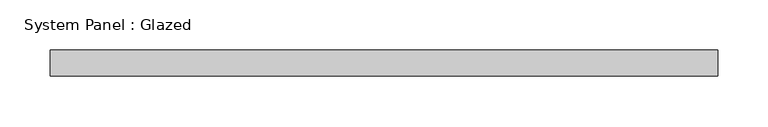
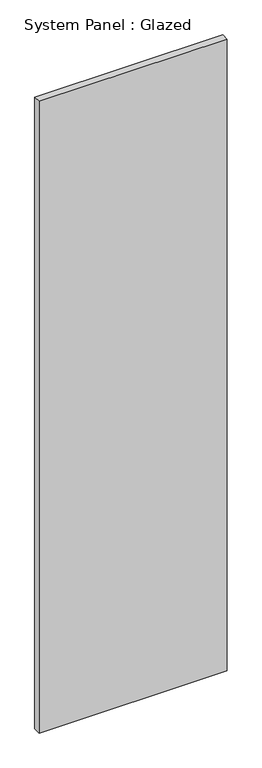
"""IFC4 building model written with IfcOpenShell, lengths in millimetres: plate geometry, System Panel : Glazed."""

from ifc_helpers import new_model, si_unit, origin, origin_with_axes, place, context, project, spatial, polyline, outline, extrude, source, transform, mapped, element, save


def system_panel_glazed_baf84a5d(model_context):
    return source(origin(), model_context, "Body", "SweptSolid", [
        extrude(outline(polyline([(330.2, -44.45), (-330.2, -44.45), (-330.2, -19.05), (330.2, -19.05), (330.2, -44.45)])), origin_with_axes(), (0.0, 0.0, 1.0), 2343.15),
    ])


if __name__ == "__main__":
    model = new_model("IFC4")
    model_context = context("Model", 3, world=origin())
    ifc_project = project(units=[si_unit("LENGTHUNIT", "METRE", prefix="MILLI")], contexts=[model_context])
    site = spatial("IfcSite", under=ifc_project)
    building = spatial("IfcBuilding", under=site)
    placement = place(None, origin())
    system_panel_glazed_shape = system_panel_glazed_baf84a5d(model_context)
    element("IfcPlate", 1, ObjectType="System Panel : Glazed", at=placement, inside=building, context=model_context, shape_type="MappedRepresentation", body=[
        mapped(system_panel_glazed_shape, transform((0.0, 0.0, 0.0), x_axis=(1.0, 0.0, 0.0), y_axis=(0.0, 1.0, 0.0), z_axis=(0.0, 0.0, 1.0))),
    ])
    save(model, "model.ifc")

# Revit data of these elements
# Type "System Panel : Glazed"
#   Construction Type Id = "GSP4R"
#   Analytic Construction = "1/8 in Pilkington single glazing"
#   Visual Light Transmittance = 0.9
#   Solar Heat Gain Coefficient = 0.86
#   Heat Transfer Coefficient (U) = 1.18115 BTU/(h·ft²·°F)
#   Define Thermal Properties by = 1
# Element 1 (IfcPlate, "System Panel : Glazed")
#   Materials on its faces: "Glass"
# Materials
#   "Glass": class "Glass", colour RGB 0 128 192, transparency 0.75, Description = "Soda Lime Glass", Cost = 0
